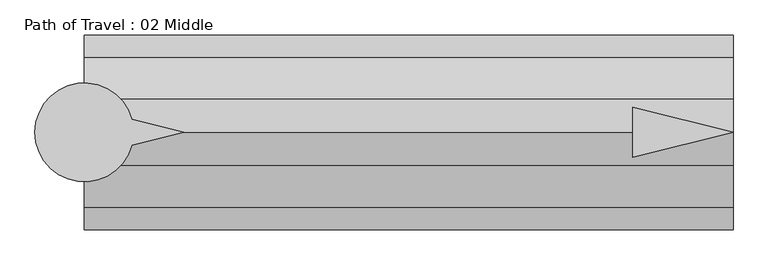
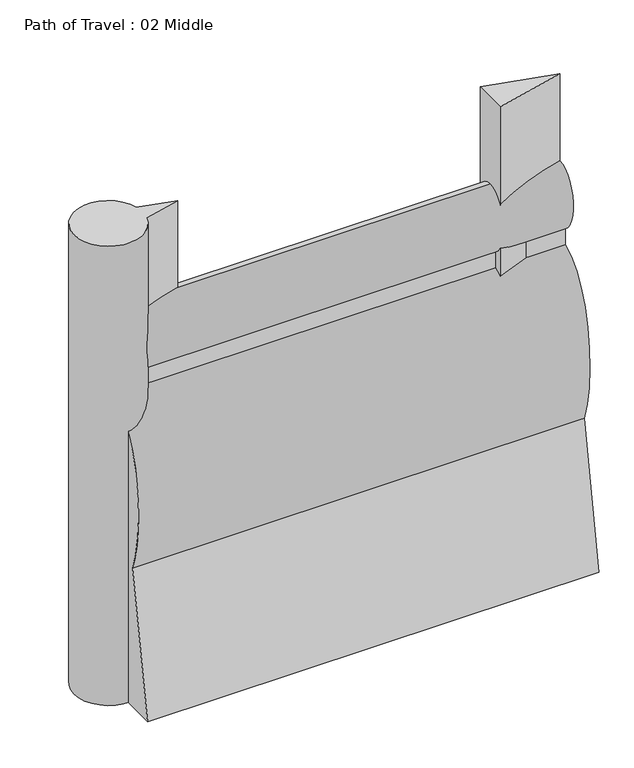
"""IFC4 building model written with IfcOpenShell, lengths in millimetres: proxy geometry, Path of Travel : 02 Middle."""

from ifc_helpers import new_model, si_unit, point, frame, frame_2d, origin, origin_with_axes, place, context, project, spatial, polyline, circle_curve, ellipse_curve, trimmed, segment, composite_curve, outline, extrude, source, transform, mapped, element, save
from ifc_brep_helpers import plane_surface, extruded_surface, advanced_brep


def path_of_travel_02_middle_3236d784(model_context):
    return source(origin(), model_context, "Body", "SolidModel", [
        advanced_brep(
        [(227.5554837, 0.0, 1727.2), (227.5554837, 42.9018657, 1436.6534209), (227.5554837, 42.9018657, 1363.4763406), (227.5554837, 184.1186263, 643.4144547), (227.5554837, 297.5699544, 0.0), (227.5554837, 145.6574193, 0.0), (227.5554837, 0.0, 584.2), (227.5554837, -145.6574193, 0.0), (227.5554837, -297.5699544, 0.0), (227.5554837, -184.1186263, 643.4144547), (227.5554837, -42.9018657, 1363.4763406), (227.5554837, -42.9018657, 1436.6534209), (2208.7554837, 0.0, 1727.2), (2208.7554837, -42.9018657, 1436.6534209), (2208.7554837, -42.9018657, 1363.4763406), (2208.7554837, -184.1186263, 643.4144547), (2208.7554837, -297.5699544, 0.0), (2208.7554837, -145.6574193, 0.0), (2208.7554837, 0.0, 584.2), (2208.7554837, 145.6574193, 0.0), (2208.7554837, 297.5699544, 0.0), (2208.7554837, 184.1186263, 643.4144547), (2208.7554837, 42.9018657, 1363.4763406), (2208.7554837, 42.9018657, 1436.6534209)],
        [
            (0, 1, ellipse_curve(frame((227.5554837, 0.0, 1574.8), z_axis=(-1.0, 0.0, 0.0), x_axis=(0.0, 0.0, 1.0)), 152.4, 101.6)),
            (1, 2),
            (2, 3, ellipse_curve(frame((227.5554837, 0.0, 914.4), z_axis=(-1.0, 0.0, 0.0), x_axis=(0.0, 0.0, -1.0)), 457.2, 228.6)),
            (3, 4),
            (4, 5),
            (5, 6),
            (6, 7),
            (7, 8),
            (8, 9),
            (9, 10, ellipse_curve(frame((227.5554837, 0.0, 914.4), z_axis=(-1.0, 0.0, 0.0), x_axis=(0.0, 0.0, -1.0)), 457.2, 228.6)),
            (10, 11),
            (11, 0, ellipse_curve(frame((227.5554837, 0.0, 1574.8), z_axis=(-1.0, 0.0, 0.0), x_axis=(0.0, 0.0, 1.0)), 152.4, 101.6)),
            (12, 13, ellipse_curve(frame((2208.7554837, 0.0, 1574.8), z_axis=(1.0, 0.0, 0.0), x_axis=(0.0, 0.0, 1.0)), 152.4, 101.6)),
            (13, 14),
            (14, 15, ellipse_curve(frame((2208.7554837, 0.0, 914.4), z_axis=(1.0, 0.0, 0.0), x_axis=(0.0, 0.0, -1.0)), 457.2, 228.6)),
            (15, 16),
            (16, 17),
            (17, 18),
            (18, 19),
            (19, 20),
            (20, 21),
            (21, 22, ellipse_curve(frame((2208.7554837, 0.0, 914.4), z_axis=(1.0, 0.0, 0.0), x_axis=(0.0, 0.0, -1.0)), 457.2, 228.6)),
            (22, 23),
            (23, 12, ellipse_curve(frame((2208.7554837, 0.0, 1574.8), z_axis=(1.0, 0.0, 0.0), x_axis=(0.0, 0.0, 1.0)), 152.4, 101.6)),
            (0, 12),
            (23, 1),
            (22, 2),
            (21, 3),
            (20, 4),
            (19, 5),
            (18, 6),
            (17, 7),
            (16, 8),
            (15, 9),
            (14, 10),
            (13, 11),
        ],
        [
            plane_surface(frame((227.5554837, 0.0, 0.0), z_axis=(-1.0, 0.0, 0.0), x_axis=(0.0, 0.0, 1.0))),
            plane_surface(frame((2208.7554837, 0.0, 0.0), z_axis=(1.0, 0.0, 0.0), x_axis=(0.0, 0.0, 1.0))),
            extruded_surface(trimmed(ellipse_curve(frame((2208.7554837, 0.0, 1574.8), z_axis=(-1.0, 0.0, 0.0), x_axis=(0.0, 0.0, 1.0)), 152.4, 101.6), [point((2208.7554837, 0.0, 1727.2))], [point((2208.7554837, 42.9018657, 1436.6534209))], True, "CARTESIAN"), (-1981.1999999999998, 0.0, 0.0), 1981.1999999999998),
            plane_surface(frame((227.5554837, 42.9018657, 1436.6534209), z_axis=(0.0, 1.0, 0.0), x_axis=(1.0, 0.0, 0.0))),
            extruded_surface(trimmed(ellipse_curve(frame((2208.7554837, 0.0, 914.4), z_axis=(-1.0, 0.0, 0.0), x_axis=(0.0, 0.0, -1.0)), 457.2, 228.6), [point((2208.7554837, 42.9018657, 1363.4763406))], [point((2208.7554837, 184.1186263, 643.4144547))], True, "CARTESIAN"), (-1981.1999999999998, 0.0, 0.0), 1981.1999999999998),
            plane_surface(frame((227.5554837, 184.1186263, 643.4144547), z_axis=(0.0, 0.9848077530122078, 0.1736481776669322), x_axis=(1.0, 0.0, 0.0))),
            plane_surface(frame((227.5554837, 297.5699544, 0.0), z_axis=(0.0, 0.0, -1.0), x_axis=(1.0, 0.0, 0.0))),
            plane_surface(frame((227.5554837, 145.6574193, 0.0), z_axis=(0.0, -0.9702957262760199, -0.2419218955995739), x_axis=(1.0, 0.0, 0.0))),
            plane_surface(frame((227.5554837, 0.0, 584.2), z_axis=(0.0, 0.9702957262759961, -0.24192189559966923), x_axis=(1.0, 0.0, 0.0))),
            plane_surface(frame((227.5554837, -145.6574193, 0.0), z_axis=(0.0, 0.0, -1.0), x_axis=(1.0, 0.0, 0.0))),
            plane_surface(frame((227.5554837, -297.5699544, 0.0), z_axis=(0.0, -0.984807753012208, 0.17364817766693066), x_axis=(1.0, 0.0, 0.0))),
            extruded_surface(trimmed(ellipse_curve(frame((2208.7554837, 0.0, 914.4), z_axis=(-1.0, 0.0, 0.0), x_axis=(0.0, 0.0, -1.0)), 457.2, 228.6), [point((2208.7554837, -184.1186263, 643.4144547))], [point((2208.7554837, -42.9018657, 1363.4763406))], True, "CARTESIAN"), (-1981.1999999999998, 0.0, 0.0), 1981.1999999999998),
            plane_surface(frame((227.5554837, -42.9018657, 1363.4763406), z_axis=(0.0, -1.0, 0.0), x_axis=(1.0, 0.0, 0.0))),
            extruded_surface(trimmed(ellipse_curve(frame((2208.7554837, 0.0, 1574.8), z_axis=(-1.0, 0.0, 0.0), x_axis=(0.0, 0.0, 1.0)), 152.4, 101.6), [point((2208.7554837, -42.9018657, 1436.6534209))], [point((2208.7554837, 0.0, 1727.2))], True, "CARTESIAN"), (-1981.1999999999998, 0.0, 0.0), 1981.1999999999998),
        ],
        [
            (0, [[1, 2, 3, 4, 5, 6, 7, 8, 9, 10, 11, 12]]),
            (1, [[13, 14, 15, 16, 17, 18, 19, 20, 21, 22, 23, 24]]),
            (2, [[-1, 25, -24, 26]]),
            (3, [[-2, -26, -23, 27]]),
            (4, [[-3, -27, -22, 28]]),
            (5, [[-4, -28, -21, 29]]),
            (6, [[-5, -29, -20, 30]]),
            (7, [[-6, -30, -19, 31]]),
            (8, [[-7, -31, -18, 32]]),
            (9, [[-8, -32, -17, 33]]),
            (10, [[-9, -33, -16, 34]]),
            (11, [[-10, -34, -15, 35]]),
            (12, [[-11, -35, -14, 36]]),
            (13, [[-12, -36, -13, -25]]),
        ],
    ),
        extrude(outline(polyline([(1902.7503371, 76.2006338), (2208.7554837, 0.0), (1902.7503371, -76.2006338), (1902.7503371, 76.2006338)])), origin_with_axes(), (0.0, 0.0, 1.0), 2129.5973753),
        extrude(outline(composite_curve([segment(polyline([(372.7837828, 39.4440225), (531.182385, 0.0), (372.7837828, -39.4440225)]), True, "CONTINUOUS"), segment(trimmed(circle_curve(frame_2d((227.2200886, 0.0)), 150.8131956), [point((372.7837828, -39.4440225))], [point((372.7837828, 39.4440225))], False, "CARTESIAN"), True, "CONTINUOUS")], self_intersect=False)), origin_with_axes(), (0.0, 0.0, 1.0), 2129.5973753),
    ])


if __name__ == "__main__":
    model = new_model("IFC4")
    model_context = context("Model", 3, world=origin())
    ifc_project = project(units=[si_unit("LENGTHUNIT", "METRE", prefix="MILLI")], contexts=[model_context])
    site = spatial("IfcSite", under=ifc_project)
    building = spatial("IfcBuilding", under=site)
    placement = place(None, origin())
    path_of_travel_02_middle_shape = path_of_travel_02_middle_3236d784(model_context)
    element("IfcBuildingElementProxy", 1, Name="Path of Travel : 02 Middle", ObjectType="Path of Travel : 02 Middle", at=placement, inside=building, context=model_context, shape_type="MappedRepresentation", body=[
        mapped(path_of_travel_02_middle_shape, transform((0.0, 0.0, 0.0), x_axis=(1.0, 0.0, 0.0), y_axis=(0.0, 1.0, 0.0), z_axis=(0.0, 0.0, 1.0))),
    ])
    save(model, "model.ifc")

# Revit data of these elements
# Type "Path of Travel : 02 Middle"
#   Path of Egress [instance default] = 4' - 0"
#   built-in parameter 1001306 [instance default] = 4 (stored number, unit not read)
#   Dot at Start = no
#   Arrow in Middle = yes
#   Arrow at End = no
#   Egress Path = none
# Element 1 (IfcBuildingElementProxy, "Path of Travel : 02 Middle")
#   Path of Egress = 6' - 6"
#   built-in parameter 1001306 = 6.5 (stored number, unit not read)
#   Materials on its faces: "Egress Path Solid", "solid"
# Materials
#   "Egress Path Solid": class "Unassigned", colour RGB 255 128 64, transparency 0.75, Comments = "Rendering appearance not upgraded "
#   "solid": class "Generic", colour RGB 120 120 120, transparency 0, Cost = 0
